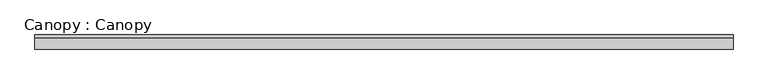
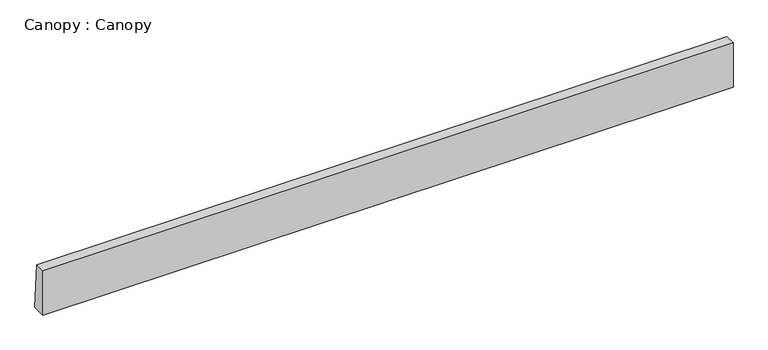
"""IFC4 building model written with IfcOpenShell, lengths in millimetres: proxy geometry, Canopy : Canopy."""

from ifc_helpers import new_model, si_unit, frame, origin, place, context, project, spatial, polyline, outline, extrude, source, transform, mapped, element, save


def canopy_canopy_990064fd(model_context):
    return source(origin(), model_context, "Body", "SweptSolid", [
        extrude(outline(polyline([(150.0, 0.0), (0.0, 0.0), (0.0, 500.0), (120.0, 500.0), (150.0, 0.0)])), frame((-3700.0, 0.0, 0.0), z_axis=(1.0, 0.0, 0.0), x_axis=(0.0, 1.0, 0.0)), (0.0, 0.0, 1.0), 7400.0),
    ])


if __name__ == "__main__":
    model = new_model("IFC4")
    model_context = context("Model", 3, world=origin())
    ifc_project = project(units=[si_unit("LENGTHUNIT", "METRE", prefix="MILLI")], contexts=[model_context])
    site = spatial("IfcSite", under=ifc_project)
    building = spatial("IfcBuilding", under=site)
    placement = place(None, origin())
    canopy_canopy_shape = canopy_canopy_990064fd(model_context)
    element("IfcBuildingElementProxy", 1, Name="Canopy : Canopy", ObjectType="Canopy : Canopy", at=placement, inside=building, context=model_context, shape_type="MappedRepresentation", body=[
        mapped(canopy_canopy_shape, transform((0.0, 0.0, 0.0), x_axis=(1.0, 0.0, 0.0), y_axis=(0.0, 1.0, 0.0), z_axis=(0.0, 0.0, 1.0))),
    ])
    save(model, "model.ifc")

# Revit data of these elements
# Type "Canopy : Canopy"
#   Type Comments = "CV-AG"
#   H_Rebar Ratio = 0.1
#   Canopy Width [instance default] = 1700 mm
#   Canopy Length [instance default] = 1000 mm
#   Canopy L.P = 120 mm
#   Canopy H.P = 150 mm
#   구조재료 = Concrete_f'c=28MPa(Cylender)
#   Default Elevation = 0
# Element 1 (IfcBuildingElementProxy, "Canopy : Canopy")
#   Canopy Width = 7400 mm
#   Canopy Length = 500 mm
#   Materials on its faces: "Concrete_f'c=28MPa(Cylender)"
# Materials
#   "Concrete_f'c=28MPa(Cylender)": class "Concrete", colour RGB 176 176 176, transparency 0, Description = "Reinf. Conc.", Cost = 0, Image = Concrete.Cast-In-Place.Flat.Polished.Grey.jpg
